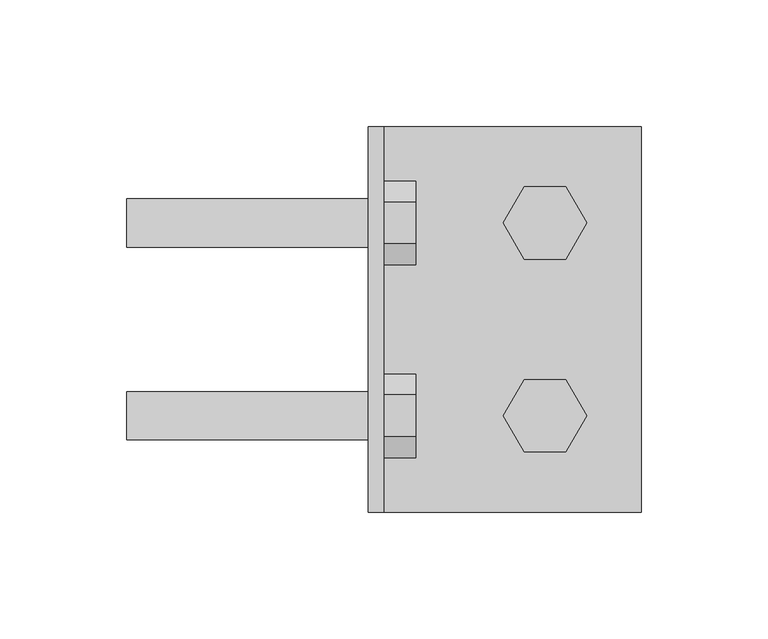
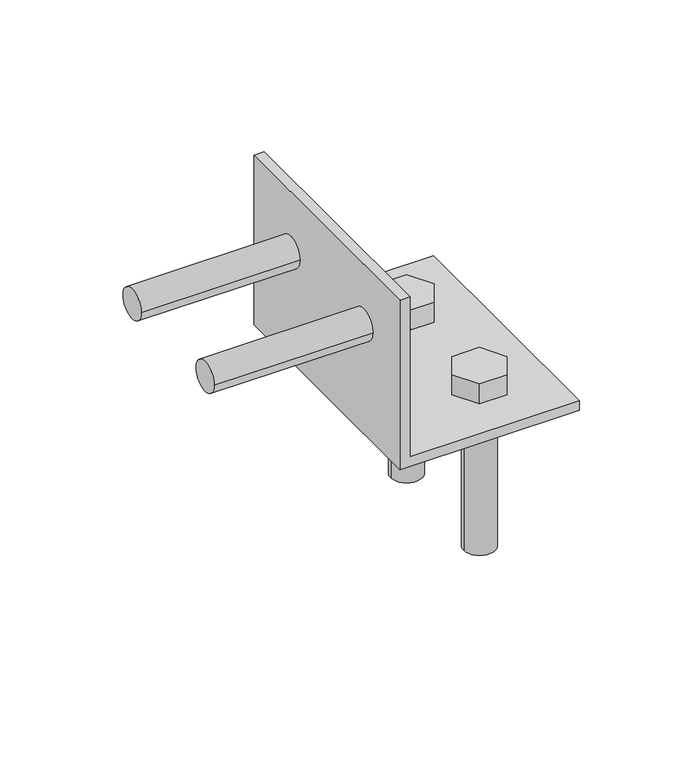
"""IFC4 building model written with IfcOpenShell, lengths in millimetres: fastener geometry, SIMPSON - HLPC/HLGPC Heavy Angles and Gussets : SIMPSON -HL46 - 6 X 4.25 - .75 Bolt - HDG."""

from ifc_helpers import new_model, si_unit, point, frame, frame_2d, origin, place, context, project, spatial, polyline, circle_curve, trimmed, segment, composite_curve, outline, extrude, source, transform, mapped, element, save
from ifc_brep_helpers import plane_surface, revolved_surface, advanced_brep


def fastener_25ec60c0(model_context):
    return source(origin(), model_context, "Body", "SolidModel", [
        extrude(outline(composite_curve([segment(trimmed(circle_curve(frame_2d((38.1, 69.85)), 9.525), [point((47.625, 69.85))], [point((28.575, 69.85))], False, "CARTESIAN"), True, "CONTINUOUS"), segment(trimmed(circle_curve(frame_2d((38.1, 69.85)), 9.525), [point((28.575, 69.85))], [point((47.625, 69.85))], False, "CARTESIAN"), True, "CONTINUOUS")], self_intersect=False)), frame((-95.5476562, 0.0, 0.0), z_axis=(1.0, 0.0, 0.0), x_axis=(0.0, 1.0, 0.0)), (0.0, 0.0, 1.0), 101.6),
        extrude(outline(polyline([(54.5977839, 69.85), (46.348892, 55.5625), (29.851108, 55.5625), (21.6022161, 69.85), (29.851108, 84.1375), (46.348892, 84.1375), (54.5977839, 69.85)])), frame((6.0523438, 0.0, 0.0), z_axis=(1.0, 0.0, 0.0), x_axis=(0.0, 1.0, 0.0)), (0.0, 0.0, 1.0), 12.7),
        extrude(outline(composite_curve([segment(trimmed(circle_curve(frame_2d((-38.1, 69.85)), 9.525), [point((-28.575, 69.85))], [point((-47.625, 69.85))], False, "CARTESIAN"), True, "CONTINUOUS"), segment(trimmed(circle_curve(frame_2d((-38.1, 69.85)), 9.525), [point((-47.625, 69.85))], [point((-28.575, 69.85))], False, "CARTESIAN"), True, "CONTINUOUS")], self_intersect=False)), frame((-95.5476562, 0.0, 0.0), z_axis=(1.0, 0.0, 0.0), x_axis=(0.0, 1.0, 0.0)), (0.0, 0.0, 1.0), 101.6),
        extrude(outline(polyline([(-21.6022161, 69.85), (-29.851108, 55.5625), (-46.348892, 55.5625), (-54.5977839, 69.85), (-46.348892, 84.1375), (-29.851108, 84.1375), (-21.6022161, 69.85)])), frame((6.0523438, 0.0, 0.0), z_axis=(1.0, 0.0, 0.0), x_axis=(0.0, 1.0, 0.0)), (0.0, 0.0, 1.0), 12.7),
        extrude(outline(composite_curve([segment(trimmed(circle_curve(frame_2d((69.85, -38.1)), 9.525), [point((60.325, -38.1))], [point((79.375, -38.1))], False, "CARTESIAN"), True, "CONTINUOUS"), segment(trimmed(circle_curve(frame_2d((69.85, -38.1)), 9.525), [point((79.375, -38.1))], [point((60.325, -38.1))], False, "CARTESIAN"), True, "CONTINUOUS")], self_intersect=False)), frame((0.0, 0.0, -95.5476563), z_axis=(0.0, 0.0, 1.0), x_axis=(1.0, 0.0, 0.0)), (0.0, 0.0, 1.0), 101.6),
        extrude(outline(polyline([(53.3522161, -38.1), (61.601108, -23.8125), (78.098892, -23.8125), (86.3477839, -38.1), (78.098892, -52.3875), (61.601108, -52.3875), (53.3522161, -38.1)])), frame((0.0, 0.0, 6.0523437), z_axis=(0.0, 0.0, 1.0), x_axis=(1.0, 0.0, 0.0)), (0.0, 0.0, 1.0), 12.7),
        extrude(outline(composite_curve([segment(trimmed(circle_curve(frame_2d((69.85, 38.1)), 9.525), [point((60.325, 38.1))], [point((79.375, 38.1))], False, "CARTESIAN"), True, "CONTINUOUS"), segment(trimmed(circle_curve(frame_2d((69.85, 38.1)), 9.525), [point((79.375, 38.1))], [point((60.325, 38.1))], False, "CARTESIAN"), True, "CONTINUOUS")], self_intersect=False)), frame((0.0, 0.0, -95.5476563), z_axis=(0.0, 0.0, 1.0), x_axis=(1.0, 0.0, 0.0)), (0.0, 0.0, 1.0), 101.6),
        extrude(outline(polyline([(53.3522161, 38.1), (61.601108, 52.3875), (78.098892, 52.3875), (86.3477839, 38.1), (78.098892, 23.8125), (61.601108, 23.8125), (53.3522161, 38.1)])), frame((0.0, 0.0, 6.0523437), z_axis=(0.0, 0.0, 1.0), x_axis=(1.0, 0.0, 0.0)), (0.0, 0.0, 1.0), 12.7),
        advanced_brep(
        [(6.0523438, -76.2, 107.95), (6.0523438, -76.2, 6.0523437), (6.0523438, 76.2, 6.0523437), (6.0523438, 76.2, 107.95), (6.0523438, 28.575, 69.85), (6.0523438, 47.625, 69.85), (6.0523438, -47.625, 69.85), (6.0523438, -28.575, 69.85), (0.0, 76.2, 107.95), (0.0, 76.2, 0.0), (0.0, -76.2, 0.0), (0.0, -76.2, 107.95), (0.0, 47.625, 69.85), (0.0, 28.575, 69.85), (0.0, -28.575, 69.85), (0.0, -47.625, 69.85), (107.95, 76.2, 6.0523437), (107.95, 76.2, 0.0), (107.95, -76.2, 0.0), (107.95, -76.2, 6.0523437), (79.375, 38.1, 6.0523437), (60.325, 38.1, 6.0523437), (79.375, -38.1, 6.0523437), (60.325, -38.1, 6.0523437), (60.325, 38.1, 0.0), (79.375, 38.1, 0.0), (60.325, -38.1, 0.0), (79.375, -38.1, 0.0)],
        [
            (0, 1),
            (1, 2),
            (2, 3),
            (3, 0),
            (4, 5, circle_curve(frame((6.0523438, 38.1, 69.85), z_axis=(-1.0, 0.0, 0.0), x_axis=(0.0, -1.0, 0.0)), 9.525)),
            (5, 4, circle_curve(frame((6.0523438, 38.1, 69.85), z_axis=(-1.0, 0.0, 0.0), x_axis=(0.0, -1.0, 0.0)), 9.525)),
            (6, 7, circle_curve(frame((6.0523438, -38.1, 69.85), z_axis=(-1.0, 0.0, 0.0), x_axis=(0.0, -1.0, 0.0)), 9.525)),
            (7, 6, circle_curve(frame((6.0523438, -38.1, 69.85), z_axis=(-1.0, 0.0, 0.0), x_axis=(0.0, -1.0, 0.0)), 9.525)),
            (8, 9),
            (9, 10),
            (10, 11),
            (11, 8),
            (12, 13, circle_curve(frame((0.0, 38.1, 69.85), z_axis=(1.0, 0.0, 0.0), x_axis=(0.0, -1.0, 0.0)), 9.525)),
            (13, 12, circle_curve(frame((0.0, 38.1, 69.85), z_axis=(1.0, 0.0, 0.0), x_axis=(0.0, -1.0, 0.0)), 9.525)),
            (14, 15, circle_curve(frame((0.0, -38.1, 69.85), z_axis=(1.0, 0.0, 0.0), x_axis=(0.0, -1.0, 0.0)), 9.525)),
            (15, 14, circle_curve(frame((0.0, -38.1, 69.85), z_axis=(1.0, 0.0, 0.0), x_axis=(0.0, -1.0, 0.0)), 9.525)),
            (3, 8),
            (11, 0),
            (2, 16),
            (16, 17),
            (17, 9),
            (10, 18),
            (18, 19),
            (19, 1),
            (19, 16),
            (20, 21, circle_curve(frame((69.85, 38.1, 6.0523437), z_axis=(0.0, 0.0, -1.0), x_axis=(1.0, 0.0, 0.0)), 9.525)),
            (21, 20, circle_curve(frame((69.85, 38.1, 6.0523437), z_axis=(0.0, 0.0, -1.0), x_axis=(1.0, 0.0, 0.0)), 9.525)),
            (22, 23, circle_curve(frame((69.85, -38.1, 6.0523437), z_axis=(0.0, 0.0, -1.0), x_axis=(1.0, 0.0, 0.0)), 9.525)),
            (23, 22, circle_curve(frame((69.85, -38.1, 6.0523437), z_axis=(0.0, 0.0, -1.0), x_axis=(1.0, 0.0, 0.0)), 9.525)),
            (17, 18),
            (24, 25, circle_curve(frame((69.85, 38.1, 0.0), z_axis=(0.0, 0.0, 1.0), x_axis=(1.0, 0.0, 0.0)), 9.525)),
            (25, 24, circle_curve(frame((69.85, 38.1, 0.0), z_axis=(0.0, 0.0, 1.0), x_axis=(1.0, 0.0, 0.0)), 9.525)),
            (26, 27, circle_curve(frame((69.85, -38.1, 0.0), z_axis=(0.0, 0.0, 1.0), x_axis=(1.0, 0.0, 0.0)), 9.525)),
            (27, 26, circle_curve(frame((69.85, -38.1, 0.0), z_axis=(0.0, 0.0, 1.0), x_axis=(1.0, 0.0, 0.0)), 9.525)),
            (21, 24),
            (25, 20),
            (23, 26),
            (27, 22),
            (5, 12),
            (13, 4),
            (7, 14),
            (15, 6),
        ],
        [
            plane_surface(frame((6.0523438, 76.2, 107.95), z_axis=(1.0, 0.0, 0.0), x_axis=(0.0, 1.0, 0.0))),
            plane_surface(frame((0.0, 76.2, 107.95), z_axis=(-1.0, 0.0, 0.0), x_axis=(0.0, -1.0, 0.0))),
            plane_surface(frame((6.0523438, -76.2, 107.95), z_axis=(0.0, 0.0, 1.0), x_axis=(-1.0, 0.0, 0.0))),
            plane_surface(frame((6.0523438, 76.2, 107.95), z_axis=(0.0, 1.0, 0.0), x_axis=(-1.0, 0.0, 0.0))),
            plane_surface(frame((6.0523438, -76.2, 6.0523437), z_axis=(0.0, -1.0, 0.0), x_axis=(-1.0, 0.0, 0.0))),
            plane_surface(frame((0.0, -76.2, 6.0523437), z_axis=(0.0, 0.0, 1.0), x_axis=(-1.0, 0.0, 0.0))),
            plane_surface(frame((0.0, -76.2, 0.0), z_axis=(0.0, 0.0, -1.0), x_axis=(1.0, 0.0, 0.0))),
            plane_surface(frame((107.95, 76.2, 6.0523437), z_axis=(1.0, 0.0, 0.0), x_axis=(0.0, 0.0, -1.0))),
            revolved_surface(polyline([(79.375, 38.1, 6.0523437), (79.375, 38.1, 0.0)]), (69.85, 38.1, 0.0), (0.0, 0.0, 1.0)),
            revolved_surface(polyline([(79.375, -38.1, 6.0523437), (79.375, -38.1, 0.0)]), (69.85, -38.1, 0.0), (0.0, 0.0, 1.0)),
            revolved_surface(polyline([(6.0523438, 28.575000000000003, 69.85), (0.0, 28.575000000000003, 69.85)]), (0.0, 38.1, 69.85), (1.0, 0.0, 0.0)),
            revolved_surface(polyline([(6.0523438, -47.625, 69.85), (0.0, -47.625, 69.85)]), (0.0, -38.1, 69.85), (1.0, 0.0, 0.0)),
        ],
        [
            (0, [[1, 2, 3, 4], [5, 6], [7, 8]]),
            (1, [[9, 10, 11, 12], [13, 14], [15, 16]]),
            (2, [[17, -12, 18, -4]]),
            (3, [[19, 20, 21, -9, -17, -3]]),
            (4, [[-18, -11, 22, 23, 24, -1]]),
            (5, [[-19, -2, -24, 25], [26, 27], [28, 29]]),
            (6, [[-22, -10, -21, 30], [31, 32], [33, 34]]),
            (7, [[-23, -30, -20, -25]]),
            (8, [[-27, 35, -32, 36]]),
            (8, [[-31, -35, -26, -36]]),
            (9, [[-29, 37, -34, 38]]),
            (9, [[-33, -37, -28, -38]]),
            (10, [[-6, 39, -14, 40]]),
            (10, [[-13, -39, -5, -40]]),
            (11, [[-8, 41, -16, 42]]),
            (11, [[-15, -41, -7, -42]]),
        ],
    ),
    ])


if __name__ == "__main__":
    model = new_model("IFC4")
    model_context = context("Model", 3, world=origin())
    ifc_project = project(units=[si_unit("LENGTHUNIT", "METRE", prefix="MILLI")], contexts=[model_context])
    site = spatial("IfcSite", under=ifc_project)
    building = spatial("IfcBuilding", under=site)
    placement = place(None, origin())
    fastener_shape = fastener_25ec60c0(model_context)
    element("IfcFastener", 1, ObjectType="SIMPSON - HLPC/HLGPC Heavy Angles and Gussets : SIMPSON -HL46 - 6 X 4.25 - .75 Bolt - HDG", at=placement, inside=building, context=model_context, shape_type="MappedRepresentation", body=[
        mapped(fastener_shape, transform((0.0, 0.0, 0.0), x_axis=(1.0, 0.0, 0.0), y_axis=(0.0, 1.0, 0.0), z_axis=(0.0, 0.0, 1.0))),
    ])
    save(model, "model.ifc")

# Revit data of these elements
# Type "SIMPSON - HLPC/HLGPC Heavy Angles and Gussets : SIMPSON -HL46 - 6 X 4.25 - .75 Bolt - HDG"
#   URL = "https://www.strongtie.com/classiccollection_architecturalproductsgroup/hlpc-hlgpc_productgroup_wcc/p/hlpc.hlgpc"
#   L = 0' - 6"
#   Hole Radius = 0' - 0 3/8"
#   D4 = 0' - 5"
#   D2 = 0' - 3"
#   D1 = 0' - 1 1/2"
#   D3 = 0' - 2 3/4"
#   Ga. = 0' - 0 61/256"
#   W1 & W2 = 0' - 4 1/4"
#   Default Elevation = 4' - 0"
#   Bolt Visibility - 3B = no
#   Bolt Visibility - 3A = no
#   Bolt Visibility - 2B = no
#   Bolt Visibility - 2A = yes
#   Bolt Visibility - 1B = no
#   Bolt Visibility - 1A = yes
#   Bolt Visibility = yes
#   Bolt Size = element 1298415
# Element 1 (IfcFastener, "SIMPSON - HLPC/HLGPC Heavy Angles and Gussets : SIMPSON -HL46 - 6 X 4.25 - .75 Bolt - HDG")
#   Materials on its faces: "1\" GALV. LAG BOLT (LENGTH = 1/2\" SHY OF GLULAM DEPTH) -  (GALV. THRU BOLT IF PLATE ON OPP. SIDE OF STRUCT MEMBER)"
# Materials
#   "1\" GALV. LAG BOLT (LENGTH = 1/2\" SHY OF GLULAM DEPTH) -  (GALV. THRU BOLT IF PLATE ON OPP. SIDE OF STRUCT MEMBER)": class "Generic", colour RGB 120 120 120, transparency 0, Cost = 0
